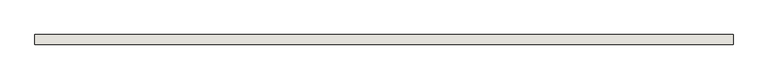
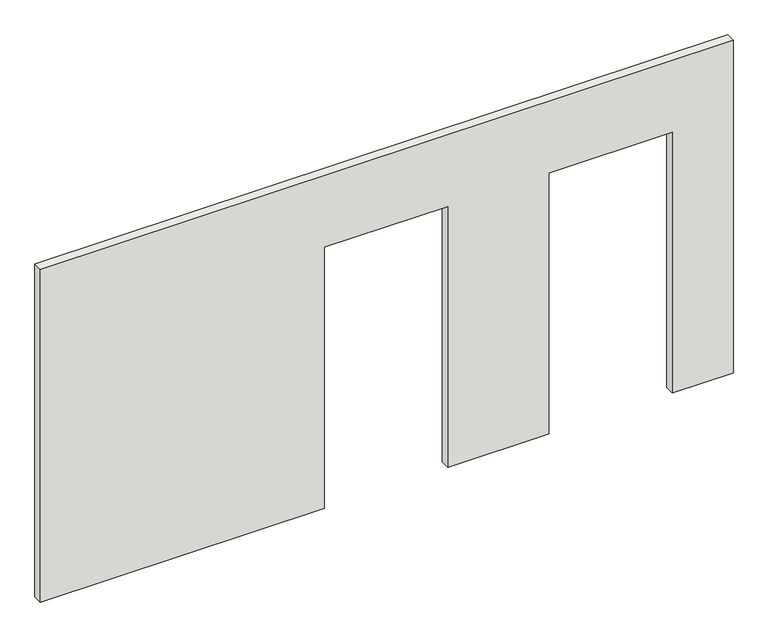
"""IFC4 building model written with IfcOpenShell, lengths in millimetres: wall geometry, 0_3d_modell."""

from ifc_helpers import new_model, si_unit, frame, origin, place, context, project, spatial, polyline, outline, extrude, source, transform, mapped, element, save


def wall_2c93ea2c(model_context):
    return source(origin(), model_context, "Body", "SweptSolid", [
        extrude(outline(polyline([(0.0, 2322.6204176), (2260.0, 2322.6204176), (2260.0, 3332.6204176), (0.0, 3332.6204176), (0.0, 4160.0), (2260.0, 4160.0), (2260.0, 5170.0), (0.0, 5170.0), (0.0, 5670.0), (2880.0, 5670.0), (2880.0, 0.0), (0.0, 0.0), (0.0, 2322.6204176)])), frame((0.0, 0.0, 0.0), z_axis=(0.0, 1.0, 0.0), x_axis=(0.0, 0.0, 1.0)), (0.0, 0.0, 1.0), 78.0),
    ])


if __name__ == "__main__":
    model = new_model("IFC4")
    model_context = context("Model", 3, world=origin())
    ifc_project = project(units=[si_unit("LENGTHUNIT", "METRE", prefix="MILLI")], contexts=[model_context])
    site = spatial("IfcSite", under=ifc_project)
    building = spatial("IfcBuilding", under=site)
    placement = place(None, origin())
    wall_shape = wall_2c93ea2c(model_context)
    element("IfcWall", 1, ObjectType="0_3d_modell", at=placement, inside=building, context=model_context, shape_type="MappedRepresentation", body=[
        mapped(wall_shape, transform((0.0, 0.0, 0.0), x_axis=(1.0, 0.0, 0.0), y_axis=(0.0, 1.0, 0.0), z_axis=(0.0, 0.0, 1.0))),
    ])
    save(model, "model.ifc")

# Revit data of these elements
# Element 1 (IfcWall, "0_3d_modell")
#   Materials on its faces: "glas"
# Materials
#   "glas": class "Unassigned", colour RGB 250 253 254, transparency 0.95
